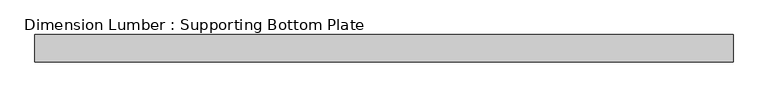
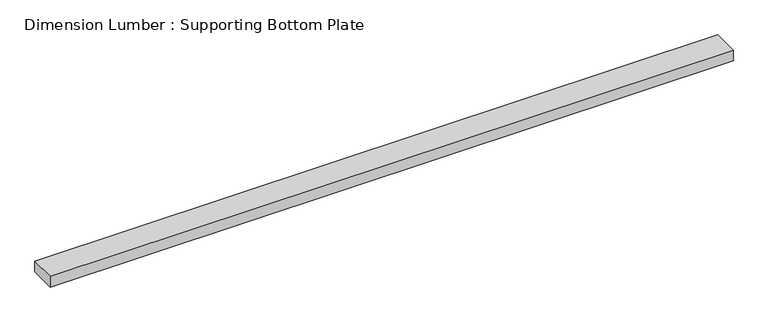
"""IFC4 building model written with IfcOpenShell, lengths in millimetres: beam geometry, Dimension Lumber : Supporting Bottom Plate."""

import ifcopenshell
import ifcopenshell.guid

model = None  # the IFC model being written
_history = None  # IfcOwnerHistory: only IFC2X3 demands one
_inside = {}  # id of a spatial element -> (the spatial element, [elements in it])
_under = {}  # id of a project, library or spatial element -> (it, [spatial elements below it])
_declared = {}  # id of a project -> (the project, [libraries it declares])
_typed = {}  # id of a type object -> (the type object, [elements of that type])
_made_of = {}  # id of a material, layer set ... -> (it, [elements and type objects made of it])


def new_model(schema):
    """Start an empty IFC model of exactly this schema.

    Asked for "IFC4X3", IfcOpenShell would pick the latest addendum, in which some entities
    have other attributes; the version numbers below select the first issue.
    IFC2X3 requires an IfcOwnerHistory on every rooted entity: one is made here for all.
    """
    global model, _history
    if schema == "IFC4X3":
        model = ifcopenshell.file(schema_version=(4, 3, 0, 0))
    else:
        model = ifcopenshell.file(schema=schema)
    _inside.clear()
    _under.clear()
    _declared.clear()
    _typed.clear()
    _made_of.clear()
    _history = None
    if model.schema == "IFC2X3":
        org = make("IfcOrganization", Name="unknown")
        user = make(
            "IfcPersonAndOrganization",
            ThePerson=make("IfcPerson", FamilyName="unknown"),
            TheOrganization=org,
        )
        app = make(
            "IfcApplication",
            ApplicationDeveloper=org,
            Version="unknown",
            ApplicationFullName="unknown",
            ApplicationIdentifier="unknown",
        )
        _history = make(
            "IfcOwnerHistory",
            OwningUser=user,
            OwningApplication=app,
            ChangeAction="ADDED",
            CreationDate=0,
        )
    return model


def make(cls, **values):
    """One entity of the class cls with the attributes given. An attribute that is None is left unset."""
    return model.create_entity(
        cls, **{name: value for name, value in values.items() if value is not None}
    )


def rooted(cls, **values):
    """An entity with a GlobalId (a new one), such as an element, a storey or a relation."""
    return make(cls, GlobalId=ifcopenshell.guid.new(), OwnerHistory=_history, **values)


def si_unit(unit_type, name, prefix=None):
    """IfcSIUnit, for example si_unit("LENGTHUNIT", "METRE", prefix="MILLI")."""
    return make("IfcSIUnit", UnitType=unit_type, Prefix=prefix, Name=name)


def assignment(units):
    """IfcUnitAssignment: the units of a project."""
    return None if units is None else make("IfcUnitAssignment", Units=units)


def point(xyz):
    """IfcCartesianPoint."""
    return None if xyz is None else make("IfcCartesianPoint", Coordinates=xyz)


def direction(xyz):
    """IfcDirection."""
    return None if xyz is None else make("IfcDirection", DirectionRatios=xyz)


def frame(location, z_axis=None, x_axis=None):
    """IfcAxis2Placement3D, a coordinate frame: its origin and axes. An axis left out is left unset."""
    return make(
        "IfcAxis2Placement3D",
        Location=point(location),
        Axis=direction(z_axis),
        RefDirection=direction(x_axis),
    )


def origin():
    """The frame at (0, 0, 0) with its axes left unset."""
    return frame((0.0, 0.0, 0.0))


def place(relative_to, where):
    """IfcLocalPlacement: puts the frame where relative to a parent placement (None: the world)."""
    return make(
        "IfcLocalPlacement", PlacementRelTo=relative_to, RelativePlacement=where
    )


def context(
    kind, dimensions, precision=None, world=None, true_north=None, identifier=None
):
    """IfcGeometricRepresentationContext, for example the 3D "Model" context."""
    return make(
        "IfcGeometricRepresentationContext",
        ContextIdentifier=identifier,
        ContextType=kind,
        CoordinateSpaceDimension=dimensions,
        Precision=precision,
        WorldCoordinateSystem=world,
        TrueNorth=true_north,
    )


def project(units=None, contexts=None):
    """IfcProject with its units and contexts."""
    return rooted(
        "IfcProject",
        Name="project",
        RepresentationContexts=contexts,
        UnitsInContext=assignment(units),
    )


def spatial(cls, under=None, at=None, **own):
    """A site, building, storey or space (cls), placed at a placement, below another one or the project."""
    s = rooted(cls, ObjectPlacement=at, **own)
    if under is not None:
        _under.setdefault(under.id(), (under, []))[1].append(s)
    return s


def polyline(points):
    """IfcPolyline through the points."""
    return make("IfcPolyline", Points=[point(p) for p in points])


def outline(outer, holes=None, kind="AREA"):
    """IfcArbitraryClosedProfileDef: a profile drawn as a closed curve; with holes, ...WithVoids."""
    if holes is None:
        return make("IfcArbitraryClosedProfileDef", ProfileType=kind, OuterCurve=outer)
    return make(
        "IfcArbitraryProfileDefWithVoids",
        ProfileType=kind,
        OuterCurve=outer,
        InnerCurves=holes,
    )


def extrude(swept, where, along, depth):
    """IfcExtrudedAreaSolid: the profile swept, set in the frame where, extruded along a direction by depth."""
    return make(
        "IfcExtrudedAreaSolid",
        SweptArea=swept,
        Position=where,
        ExtrudedDirection=direction(along),
        Depth=depth,
    )


def shape(context_of_items, identifier, shape_type, items):
    """IfcShapeRepresentation: the items that make up one representation, for example the "Body"."""
    return make(
        "IfcShapeRepresentation",
        ContextOfItems=context_of_items,
        RepresentationIdentifier=identifier,
        RepresentationType=shape_type,
        Items=items,
    )


def source(mapping_origin, context_of_items, identifier, shape_type, items):
    """IfcRepresentationMap: a shape defined once, which mapped items show again and again."""
    return make(
        "IfcRepresentationMap",
        MappingOrigin=mapping_origin,
        MappedRepresentation=shape(context_of_items, identifier, shape_type, items),
    )


def transform(
    local_origin,
    x_axis=None,
    y_axis=None,
    z_axis=None,
    scale=None,
    scale2=None,
    scale3=None,
    uniform=True,
):
    """IfcCartesianTransformationOperator3D, or its non-uniform kind. x_axis, y_axis, z_axis: its Axis1, 2, 3."""
    if uniform:
        return make(
            "IfcCartesianTransformationOperator3D",
            Axis1=direction(x_axis),
            Axis2=direction(y_axis),
            LocalOrigin=point(local_origin),
            Scale=scale,
            Axis3=direction(z_axis),
        )
    return make(
        "IfcCartesianTransformationOperator3DnonUniform",
        Axis1=direction(x_axis),
        Axis2=direction(y_axis),
        LocalOrigin=point(local_origin),
        Scale=scale,
        Axis3=direction(z_axis),
        Scale2=scale2,
        Scale3=scale3,
    )


def mapped(mapping_source, mapping_target):
    """IfcMappedItem: shows the shape of a source again, moved by a transform."""
    return make(
        "IfcMappedItem", MappingSource=mapping_source, MappingTarget=mapping_target
    )


def made_of(thing, what):
    """Note that an element or type object is made of a material, layer set ...; save() writes the relation."""
    if what is not None:
        _made_of.setdefault(what.id(), (what, []))[1].append(thing)
    return thing


def element(
    cls,
    number,
    at=None,
    inside=None,
    cuts=None,
    type_object=None,
    material=None,
    context=None,
    identifier="Body",
    shape_type=None,
    held_by="IfcProductDefinitionShape",
    body=None,
    shapes=None,
    **own,
):
    """One element of the class cls, such as IfcWall. Its Tag is "e" and its number.

    at: its placement. inside: the storey or other place that contains it. cuts: it is an
    opening in that element (IfcRelVoidsElement). A single representation is given by context,
    identifier, shape_type and body (its items); several are given by shapes. held_by: the class
    of the entity that holds the representations. save() writes the other relations.
    """
    e = rooted(cls, Tag="e%d" % number, ObjectPlacement=at, **own)
    if body is not None:
        shapes = [shape(context, identifier, shape_type, body)]
    if shapes is not None:
        e.Representation = make(held_by, Representations=shapes)
    if inside is not None:
        _inside.setdefault(inside.id(), (inside, []))[1].append(e)
    if cuts is not None:
        rooted(
            "IfcRelVoidsElement", RelatingBuildingElement=cuts, RelatedOpeningElement=e
        )
    if type_object is not None:
        _typed.setdefault(type_object.id(), (type_object, []))[1].append(e)
    return made_of(e, material)


def aggregate(whole, parts):
    """IfcRelAggregates: a whole, such as a stair, and the parts it consists of."""
    return rooted("IfcRelAggregates", RelatingObject=whole, RelatedObjects=parts)


def save(model, path):
    """Write the relations noted so far, then the file.

    IfcRelAggregates (storeys below a building ...), IfcRelContainedInSpatialStructure (elements
    in a storey), IfcRelDefinesByType, IfcRelAssociatesMaterial and IfcRelDeclares: one each for
    every whole, place, type object, material and project.
    """
    for whole, parts in _under.values():
        aggregate(whole, parts)
    for where, things in _inside.values():
        rooted(
            "IfcRelContainedInSpatialStructure",
            RelatedElements=things,
            RelatingStructure=where,
        )
    for kind, things in _typed.values():
        rooted("IfcRelDefinesByType", RelatedObjects=things, RelatingType=kind)
    for what, things in _made_of.values():
        rooted("IfcRelAssociatesMaterial", RelatedObjects=things, RelatingMaterial=what)
    for by, libraries in _declared.values():
        rooted("IfcRelDeclares", RelatingContext=by, RelatedDefinitions=libraries)
    model.write(path)


def dimension_lumber_supporting_bottom_plate_fd513b8e(model_context):
    return source(origin(), model_context, "Body", "SweptSolid", [
        extrude(outline(polyline([(1118.39375, 44.45), (1118.39375, -44.45), (-1165.225, -44.45), (-1165.225, 44.45), (1118.39375, 44.45)])), frame((0.0, 0.0, -19.05), z_axis=(0.0, 0.0, 1.0), x_axis=(1.0, 0.0, 0.0)), (0.0, 0.0, 1.0), 38.1),
    ])


if __name__ == "__main__":
    model = new_model("IFC4")
    model_context = context("Model", 3, world=origin())
    ifc_project = project(units=[si_unit("LENGTHUNIT", "METRE", prefix="MILLI")], contexts=[model_context])
    site = spatial("IfcSite", under=ifc_project)
    building = spatial("IfcBuilding", under=site)
    placement = place(None, origin())
    dimension_lumber_supporting_bottom_plate_shape = dimension_lumber_supporting_bottom_plate_fd513b8e(model_context)
    element("IfcBeam", 1, ObjectType="Dimension Lumber : Supporting Bottom Plate", at=placement, inside=building, context=model_context, shape_type="MappedRepresentation", body=[
        mapped(dimension_lumber_supporting_bottom_plate_shape, transform((0.0, 0.0, 0.0), x_axis=(1.0, 0.0, 0.0), y_axis=(0.0, 1.0, 0.0), z_axis=(0.0, 0.0, 1.0))),
    ])
    save(model, "model.ifc")

# Revit data of these elements
# Type "Dimension Lumber : Supporting Bottom Plate"
#   Assembly Code = "B10"
#   A = 0.0364583 SF
#   Length [instance default] = 5' - 0"
#   b = 0' - 3 1/2"
#   d = 0' - 1 1/2"
#   Structural Material [instance default] = Softwood, Lumber
# Element 1 (IfcBeam, "Dimension Lumber : Supporting Bottom Plate")
#   Structural Material = Douglas Fir #2
#   Materials on its faces: "Douglas Fir #2"
# Materials
#   "Softwood, Lumber": class "Wood", colour RGB 223 192 134, transparency 0, Description = "Pinus Echinata", Cost = 0
#   "Douglas Fir #2": class "Wood", colour RGB 223 192 134, transparency 0, Description = "Pinus Echinata", Cost = 0
